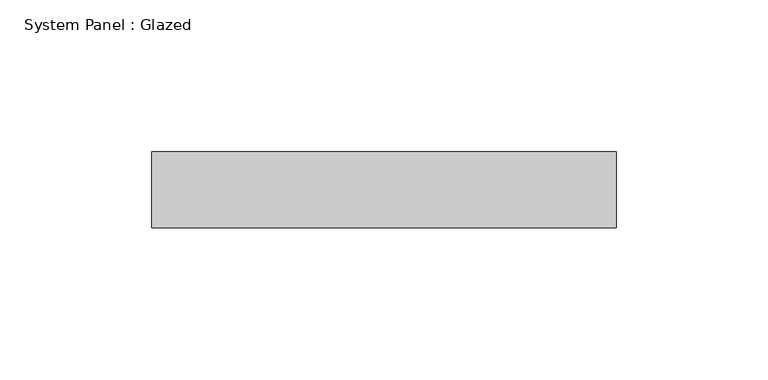
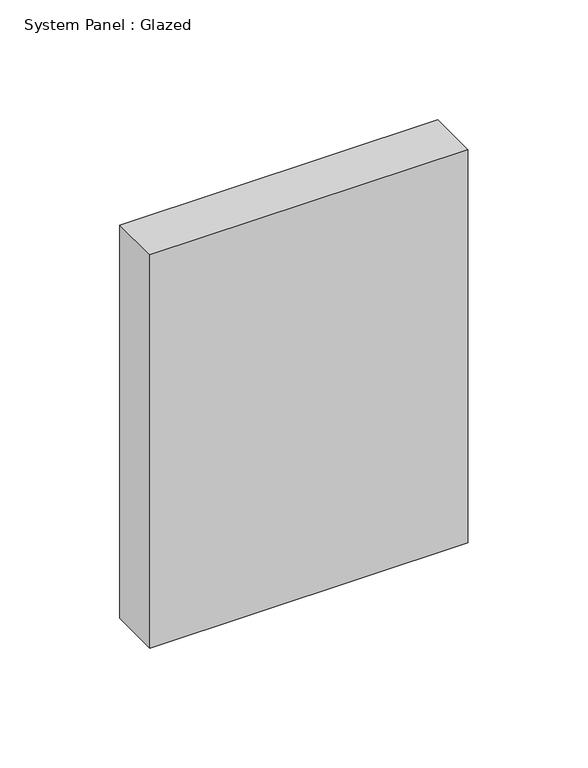
"""IFC4 building model written with IfcOpenShell, lengths in millimetres: plate geometry, System Panel : Glazed."""

from ifc_helpers import new_model, si_unit, origin, origin_with_axes, place, context, project, spatial, polyline, outline, extrude, source, transform, mapped, element, save


def system_panel_glazed_2f597917(model_context):
    return source(origin(), model_context, "Body", "SweptSolid", [
        extrude(outline(polyline([(76.4636532, 24.5), (-76.4636532, 24.5), (-76.4636532, 49.5), (76.4636532, 49.5), (76.4636532, 24.5)])), origin_with_axes(), (0.0, 0.0, 1.0), 200.0),
    ])


if __name__ == "__main__":
    model = new_model("IFC4")
    model_context = context("Model", 3, world=origin())
    ifc_project = project(units=[si_unit("LENGTHUNIT", "METRE", prefix="MILLI")], contexts=[model_context])
    site = spatial("IfcSite", under=ifc_project)
    building = spatial("IfcBuilding", under=site)
    placement = place(None, origin())
    system_panel_glazed_shape = system_panel_glazed_2f597917(model_context)
    element("IfcPlate", 1, ObjectType="System Panel : Glazed", at=placement, inside=building, context=model_context, shape_type="MappedRepresentation", body=[
        mapped(system_panel_glazed_shape, transform((0.0, 0.0, 0.0), x_axis=(1.0, 0.0, 0.0), y_axis=(0.0, 1.0, 0.0), z_axis=(0.0, 0.0, 1.0))),
    ])
    save(model, "model.ifc")

# Revit data of these elements
# Element 1 (IfcPlate, "System Panel : Glazed")
#   Materials on its faces: "Glass"
# Materials
#   "Glass": class "Glass", colour RGB 218 227 224, transparency 0.85, Description = "Soda Lime Glass", Cost = 0
